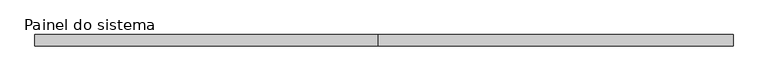
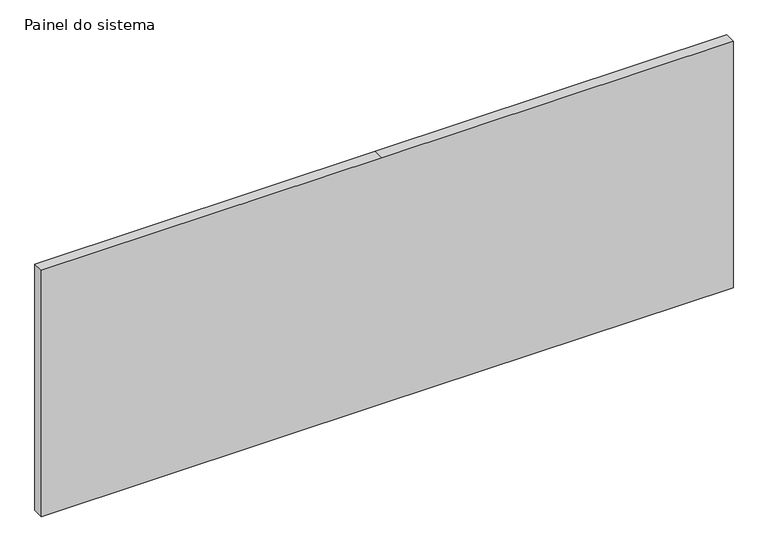
"""IFC4 building model written with IfcOpenShell, lengths in millimetres: plate geometry, Painel do sistema : Envidraçado."""

import ifcopenshell
import ifcopenshell.guid

model = None  # the IFC model being written
_history = None  # IfcOwnerHistory: only IFC2X3 demands one
_inside = {}  # id of a spatial element -> (the spatial element, [elements in it])
_under = {}  # id of a project, library or spatial element -> (it, [spatial elements below it])
_declared = {}  # id of a project -> (the project, [libraries it declares])
_typed = {}  # id of a type object -> (the type object, [elements of that type])
_made_of = {}  # id of a material, layer set ... -> (it, [elements and type objects made of it])


def new_model(schema):
    """Start an empty IFC model of exactly this schema.

    Asked for "IFC4X3", IfcOpenShell would pick the latest addendum, in which some entities
    have other attributes; the version numbers below select the first issue.
    IFC2X3 requires an IfcOwnerHistory on every rooted entity: one is made here for all.
    """
    global model, _history
    if schema == "IFC4X3":
        model = ifcopenshell.file(schema_version=(4, 3, 0, 0))
    else:
        model = ifcopenshell.file(schema=schema)
    _inside.clear()
    _under.clear()
    _declared.clear()
    _typed.clear()
    _made_of.clear()
    _history = None
    if model.schema == "IFC2X3":
        org = make("IfcOrganization", Name="unknown")
        user = make(
            "IfcPersonAndOrganization",
            ThePerson=make("IfcPerson", FamilyName="unknown"),
            TheOrganization=org,
        )
        app = make(
            "IfcApplication",
            ApplicationDeveloper=org,
            Version="unknown",
            ApplicationFullName="unknown",
            ApplicationIdentifier="unknown",
        )
        _history = make(
            "IfcOwnerHistory",
            OwningUser=user,
            OwningApplication=app,
            ChangeAction="ADDED",
            CreationDate=0,
        )
    return model


def make(cls, **values):
    """One entity of the class cls with the attributes given. An attribute that is None is left unset."""
    return model.create_entity(
        cls, **{name: value for name, value in values.items() if value is not None}
    )


def rooted(cls, **values):
    """An entity with a GlobalId (a new one), such as an element, a storey or a relation."""
    return make(cls, GlobalId=ifcopenshell.guid.new(), OwnerHistory=_history, **values)


def si_unit(unit_type, name, prefix=None):
    """IfcSIUnit, for example si_unit("LENGTHUNIT", "METRE", prefix="MILLI")."""
    return make("IfcSIUnit", UnitType=unit_type, Prefix=prefix, Name=name)


def assignment(units):
    """IfcUnitAssignment: the units of a project."""
    return None if units is None else make("IfcUnitAssignment", Units=units)


def point(xyz):
    """IfcCartesianPoint."""
    return None if xyz is None else make("IfcCartesianPoint", Coordinates=xyz)


def direction(xyz):
    """IfcDirection."""
    return None if xyz is None else make("IfcDirection", DirectionRatios=xyz)


def frame(location, z_axis=None, x_axis=None):
    """IfcAxis2Placement3D, a coordinate frame: its origin and axes. An axis left out is left unset."""
    return make(
        "IfcAxis2Placement3D",
        Location=point(location),
        Axis=direction(z_axis),
        RefDirection=direction(x_axis),
    )


def origin():
    """The frame at (0, 0, 0) with its axes left unset."""
    return frame((0.0, 0.0, 0.0))


def place(relative_to, where):
    """IfcLocalPlacement: puts the frame where relative to a parent placement (None: the world)."""
    return make(
        "IfcLocalPlacement", PlacementRelTo=relative_to, RelativePlacement=where
    )


def context(
    kind, dimensions, precision=None, world=None, true_north=None, identifier=None
):
    """IfcGeometricRepresentationContext, for example the 3D "Model" context."""
    return make(
        "IfcGeometricRepresentationContext",
        ContextIdentifier=identifier,
        ContextType=kind,
        CoordinateSpaceDimension=dimensions,
        Precision=precision,
        WorldCoordinateSystem=world,
        TrueNorth=true_north,
    )


def project(units=None, contexts=None):
    """IfcProject with its units and contexts."""
    return rooted(
        "IfcProject",
        Name="project",
        RepresentationContexts=contexts,
        UnitsInContext=assignment(units),
    )


def spatial(cls, under=None, at=None, **own):
    """A site, building, storey or space (cls), placed at a placement, below another one or the project."""
    s = rooted(cls, ObjectPlacement=at, **own)
    if under is not None:
        _under.setdefault(under.id(), (under, []))[1].append(s)
    return s


def polyline(points):
    """IfcPolyline through the points."""
    return make("IfcPolyline", Points=[point(p) for p in points])


def outline(outer, holes=None, kind="AREA"):
    """IfcArbitraryClosedProfileDef: a profile drawn as a closed curve; with holes, ...WithVoids."""
    if holes is None:
        return make("IfcArbitraryClosedProfileDef", ProfileType=kind, OuterCurve=outer)
    return make(
        "IfcArbitraryProfileDefWithVoids",
        ProfileType=kind,
        OuterCurve=outer,
        InnerCurves=holes,
    )


def extrude(swept, where, along, depth):
    """IfcExtrudedAreaSolid: the profile swept, set in the frame where, extruded along a direction by depth."""
    return make(
        "IfcExtrudedAreaSolid",
        SweptArea=swept,
        Position=where,
        ExtrudedDirection=direction(along),
        Depth=depth,
    )


def shape(context_of_items, identifier, shape_type, items):
    """IfcShapeRepresentation: the items that make up one representation, for example the "Body"."""
    return make(
        "IfcShapeRepresentation",
        ContextOfItems=context_of_items,
        RepresentationIdentifier=identifier,
        RepresentationType=shape_type,
        Items=items,
    )


def source(mapping_origin, context_of_items, identifier, shape_type, items):
    """IfcRepresentationMap: a shape defined once, which mapped items show again and again."""
    return make(
        "IfcRepresentationMap",
        MappingOrigin=mapping_origin,
        MappedRepresentation=shape(context_of_items, identifier, shape_type, items),
    )


def transform(
    local_origin,
    x_axis=None,
    y_axis=None,
    z_axis=None,
    scale=None,
    scale2=None,
    scale3=None,
    uniform=True,
):
    """IfcCartesianTransformationOperator3D, or its non-uniform kind. x_axis, y_axis, z_axis: its Axis1, 2, 3."""
    if uniform:
        return make(
            "IfcCartesianTransformationOperator3D",
            Axis1=direction(x_axis),
            Axis2=direction(y_axis),
            LocalOrigin=point(local_origin),
            Scale=scale,
            Axis3=direction(z_axis),
        )
    return make(
        "IfcCartesianTransformationOperator3DnonUniform",
        Axis1=direction(x_axis),
        Axis2=direction(y_axis),
        LocalOrigin=point(local_origin),
        Scale=scale,
        Axis3=direction(z_axis),
        Scale2=scale2,
        Scale3=scale3,
    )


def mapped(mapping_source, mapping_target):
    """IfcMappedItem: shows the shape of a source again, moved by a transform."""
    return make(
        "IfcMappedItem", MappingSource=mapping_source, MappingTarget=mapping_target
    )


def made_of(thing, what):
    """Note that an element or type object is made of a material, layer set ...; save() writes the relation."""
    if what is not None:
        _made_of.setdefault(what.id(), (what, []))[1].append(thing)
    return thing


def element(
    cls,
    number,
    at=None,
    inside=None,
    cuts=None,
    type_object=None,
    material=None,
    context=None,
    identifier="Body",
    shape_type=None,
    held_by="IfcProductDefinitionShape",
    body=None,
    shapes=None,
    **own,
):
    """One element of the class cls, such as IfcWall. Its Tag is "e" and its number.

    at: its placement. inside: the storey or other place that contains it. cuts: it is an
    opening in that element (IfcRelVoidsElement). A single representation is given by context,
    identifier, shape_type and body (its items); several are given by shapes. held_by: the class
    of the entity that holds the representations. save() writes the other relations.
    """
    e = rooted(cls, Tag="e%d" % number, ObjectPlacement=at, **own)
    if body is not None:
        shapes = [shape(context, identifier, shape_type, body)]
    if shapes is not None:
        e.Representation = make(held_by, Representations=shapes)
    if inside is not None:
        _inside.setdefault(inside.id(), (inside, []))[1].append(e)
    if cuts is not None:
        rooted(
            "IfcRelVoidsElement", RelatingBuildingElement=cuts, RelatedOpeningElement=e
        )
    if type_object is not None:
        _typed.setdefault(type_object.id(), (type_object, []))[1].append(e)
    return made_of(e, material)


def aggregate(whole, parts):
    """IfcRelAggregates: a whole, such as a stair, and the parts it consists of."""
    return rooted("IfcRelAggregates", RelatingObject=whole, RelatedObjects=parts)


def save(model, path):
    """Write the relations noted so far, then the file.

    IfcRelAggregates (storeys below a building ...), IfcRelContainedInSpatialStructure (elements
    in a storey), IfcRelDefinesByType, IfcRelAssociatesMaterial and IfcRelDeclares: one each for
    every whole, place, type object, material and project.
    """
    for whole, parts in _under.values():
        aggregate(whole, parts)
    for where, things in _inside.values():
        rooted(
            "IfcRelContainedInSpatialStructure",
            RelatedElements=things,
            RelatingStructure=where,
        )
    for kind, things in _typed.values():
        rooted("IfcRelDefinesByType", RelatedObjects=things, RelatingType=kind)
    for what, things in _made_of.values():
        rooted("IfcRelAssociatesMaterial", RelatedObjects=things, RelatingMaterial=what)
    for by, libraries in _declared.values():
        rooted("IfcRelDeclares", RelatingContext=by, RelatedDefinitions=libraries)
    model.write(path)


def painel_do_sistema_d52e1df4(model_context):
    return source(origin(), model_context, "Body", "SweptSolid", [
        extrude(outline(polyline([(0.0, -783.4833334), (0.0, -12.4999998), (0.0, 783.4833334), (590.0, 783.4833334), (590.0, -12.4999998), (590.0, -783.4833334), (0.0, -783.4833334)])), frame((0.0, -49.5, 0.0), z_axis=(0.0, 1.0, 0.0), x_axis=(0.0, 0.0, 1.0)), (0.0, 0.0, 1.0), 25.0),
    ])


if __name__ == "__main__":
    model = new_model("IFC4")
    model_context = context("Model", 3, world=origin())
    ifc_project = project(units=[si_unit("LENGTHUNIT", "METRE", prefix="MILLI")], contexts=[model_context])
    site = spatial("IfcSite", under=ifc_project)
    building = spatial("IfcBuilding", under=site)
    placement = place(None, origin())
    painel_do_sistema_shape = painel_do_sistema_d52e1df4(model_context)
    element("IfcPlate", 1, ObjectType="Painel do sistema : Envidraçado", at=placement, inside=building, context=model_context, shape_type="MappedRepresentation", body=[
        mapped(painel_do_sistema_shape, transform((0.0, 0.0, 0.0), x_axis=(1.0, 0.0, 0.0), y_axis=(0.0, 1.0, 0.0), z_axis=(0.0, 0.0, 1.0))),
    ])
    save(model, "model.ifc")

# Revit data of these elements
# Type "Painel do sistema : Envidraçado"
#   Construction Type Id = "GSP4R"
#   Analytic Construction = "Vidraça única Pilkington 1/8 pol"
#   Visual Light Transmittance = 0.9
#   Solar Heat Gain Coefficient = 0.86
#   Heat Transfer Coefficient (U) = 6.7069 W/(m²·K)
# Element 1 (IfcPlate, "Painel do sistema : Envidraçado")
#   Materials on its faces: ".VIDRO GENÉRICO"
# Materials
#   ".VIDRO GENÉRICO": class ".CC_VIDRO", colour RGB 0 128 192, transparency 0.9, Description = "Vidro comum", Cost = 0
